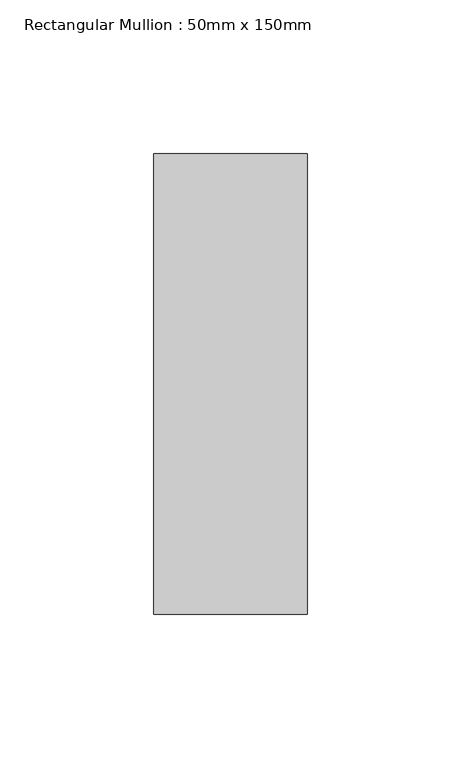
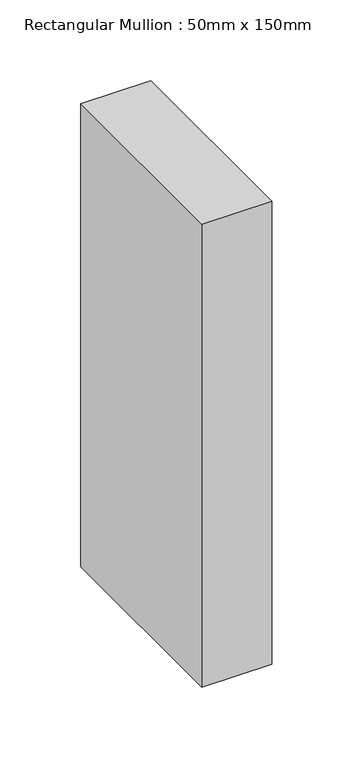
"""IFC4 building model written with IfcOpenShell, lengths in millimetres: member geometry, Rectangular Mullion : 50mm x 150mm."""

from ifc_helpers import new_model, si_unit, frame, origin, place, context, project, spatial, polyline, outline, extrude, source, transform, mapped, element, save


def rectangular_mullion_50mm_x_150mm_23485ade(model_context):
    return source(origin(), model_context, "Body", "SweptSolid", [
        extrude(outline(polyline([(0.0, 75.0), (0.0, -75.0), (-50.0, -75.0), (-50.0, 75.0), (0.0, 75.0)])), frame((0.0, 0.0, -350.0), z_axis=(0.0, 0.0, 1.0), x_axis=(1.0, 0.0, 0.0)), (0.0, 0.0, 1.0), 350.0),
    ])


if __name__ == "__main__":
    model = new_model("IFC4")
    model_context = context("Model", 3, world=origin())
    ifc_project = project(units=[si_unit("LENGTHUNIT", "METRE", prefix="MILLI")], contexts=[model_context])
    site = spatial("IfcSite", under=ifc_project)
    building = spatial("IfcBuilding", under=site)
    placement = place(None, origin())
    rectangular_mullion_50mm_x_150mm_shape = rectangular_mullion_50mm_x_150mm_23485ade(model_context)
    element("IfcMember", 1, ObjectType="Rectangular Mullion : 50mm x 150mm", at=placement, inside=building, context=model_context, shape_type="MappedRepresentation", body=[
        mapped(rectangular_mullion_50mm_x_150mm_shape, transform((0.0, 0.0, 0.0), x_axis=(1.0, 0.0, 0.0), y_axis=(0.0, 1.0, 0.0), z_axis=(0.0, 0.0, 1.0))),
    ])
    save(model, "model.ifc")

# Revit data of these elements
# Type "Rectangular Mullion : 50mm x 150mm"
#   built-in parameter 1007304 = 0.492126 (stored number, unit not read)
#   built-in parameter 1007301 = 0.082021 (stored number, unit not read)
#   built-in parameter 1007300 = 0.082021 (stored number, unit not read)
# Element 1 (IfcMember, "Rectangular Mullion : 50mm x 150mm")
#   Materials on its faces: "Aluminum"
# Materials
#   "Aluminum": class "Metal", colour RGB 244 244 244, transparency 0, Description = "Aluminum 6061", Cost = 0
